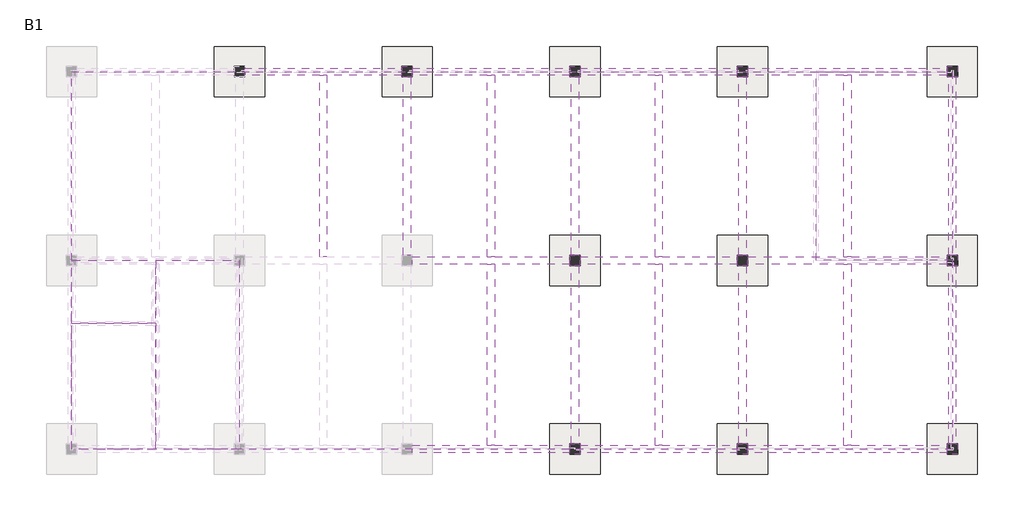
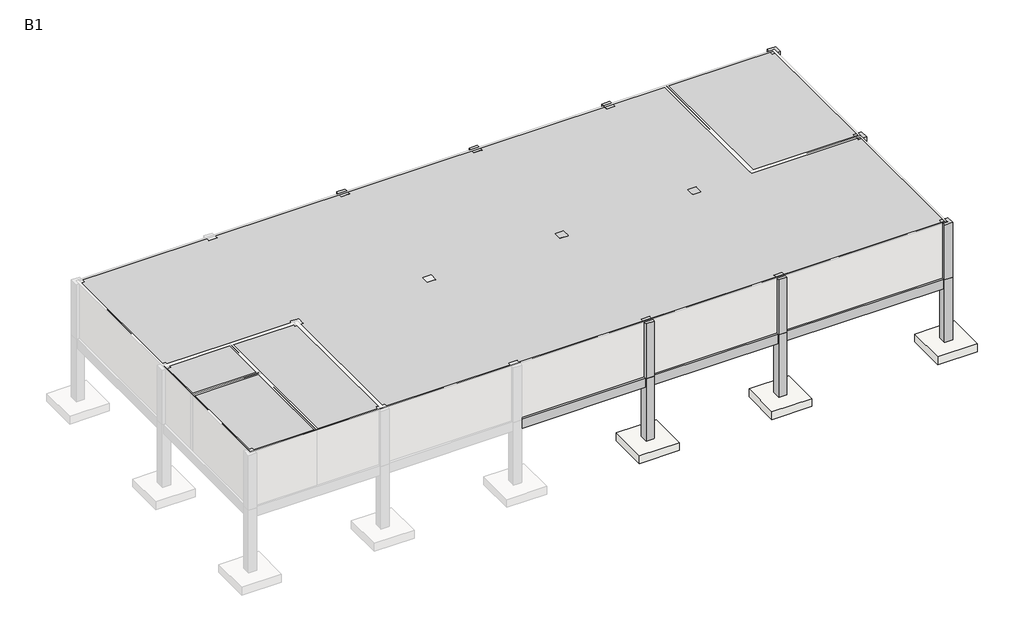
# One storey, part 2 of 2: 24 beams, 21 columns, 11 slabs, 5 proxies.
# Revit data of these elements (continued)
# Element 27 (IfcBuildingElementProxy, "Space Planning Box_hec : Space Planning Box_hec") (continued)
#   Interior Finish = "IW5..N/A..N/A,,WK3..N/A,,FL2..N/A,,N/A..N/A"
#   Exterior Finish = "N/A..N/A,,EW2..N/A..N/A"
#   Department = "AR"
#   ceiling height = 0
#   Width = 4000 mm
#   Program Area = 0.00 m²
#   Length = 9000 mm
#   Height = 3500 mm
#   Area = 36.00 m²
#   Fill Color = Cyan
#   Phase Created = New Construction
#   Materials on its faces: "Cyan"
# Element 28 (IfcBuildingElementProxy, "Space Planning Box_hec : Space Planning Box_hec")
#   Room Name = "Elevator"
#   Interior Finish = "N/A..N/A..N/A,,N/A..N/A,,,,CL3..N/A"
#   Exterior Finish = "N/A..N/A,,EW2..N/A..N/A"
#   Department = "AR"
#   ceiling height = 0
#   Width = 4000 mm
#   Program Area = 0.00 m²
#   Length = 3000 mm
#   Height = 3500 mm
#   Area = 12.00 m²
#   Fill Color = Cyan
#   Phase Created = New Construction
#   Materials on its faces: "Cyan"
# Element 29 (IfcBuildingElementProxy, "Space Planning Box_hec : Space Planning Box_hec")
#   Room Name = "Stairway"
#   Interior Finish = "IW5..N/A..N/A,,WK3..N/A,,FL2..N/A,,CL1..N/A"
#   Exterior Finish = "N/A..N/A,,EW2..N/A..N/A"
#   Department = "PATHV1"
#   ceiling height = 0
#   Width = 4000 mm
#   Program Area = 36.00 m²
#   Length = 6000 mm
#   Height = 3500 mm
#   Area = 24.00 m²
#   Fill Color = Green
#   Phase Created = New Construction
#   Materials on its faces: "Green"
# Elements 30, 31, 32, 33, 34, 35, 36, 37, 38, 39, 40, 41, 42, 43, 44, 45, 46, 47, 48, 49, 50 (IfcColumn, "Concrete-Rectangular-Column : CL111_500x500")
#   Comments = ""
#   hec_material3 = none
#   hec_material2 = none
#   hec_material1 = none
#   Structural Material = 콘크리트 - 현장타설 콘크리트
#   Phase Created = New Construction
#   Materials on its faces: "콘크리트 - 현장타설 콘크리트"
# Elements 51, 52, 53, 54, 55, 56, 57, 58, 59, 60, 61 (IfcSlab, "FT112-Footing-Rectangular : FT112_2400x2400x500")
#   Comments = ""
#   hec_material3 = none
#   hec_material2 = none
#   hec_material1 = none
#   Structural Material = 콘크리트 - 현장타설 콘크리트
#   Phase Created = New Construction
#   Materials on its faces: "콘크리트 - 현장타설 콘크리트"
# Materials
#   "콘크리트 - 현장타설 콘크리트": class "콘크리트", colour RGB 192 192 192, transparency 0
#   "Cyan": class "Generic", colour RGB 0 255 255, transparency 0.2, Cost = 0
#   "A03AE056-00001_Bitumen/Bituminous/Asphalt Coating": class "Generic", colour RGB 17 17 17, transparency 0, Description = "Damp-proofing", W00) Work Master Code = "A03AE056-00001", W01) Work Master_Lv1 = "Concrete Work", W02) Work Master_Lv2 = "Concrete Protective Coating (U/G)", W03) Work Master_Spec.1 = "Bitumen/Bituminous/Asphalt Coating", Cost = 0
#   "A03AC035-00001_Form Work (3 times in use)_Flat": class "Wood", colour RGB 149 120 74, transparency 0, Description = "Plywood", W00) Work Master Code = "A03AC035-00001", W01) Work Master_Lv1 = "Concrete Work", W02) Work Master_Lv2 = "Substructure Work", W03) Work Master_Spec.1 = "Form Work (3 times in use)", W04) Work Master_Spec.2 = "Flat Form", W05) Work Master_Spec.3 = "Dressed Lumber, Plywood or Steel Form(Wood Planks are not Allowed) incl. Chamfer", Cost = 0
#   "A03AC032-00007_Structural Concrete_Type1_25MPa-30Mpa": class "Concrete", colour RGB 176 176 176, transparency 0, Keynote = "09910.A1", Description = "Reinf. Conc.", W00) Work Master Code = "A03AC032-00007", W01) Work Master_Lv1 = "Concrete Work", W02) Work Master_Lv2 = "Substructure Work", W03) Work Master_Spec.1 = "Structural Concrete", W04) Work Master_Spec.2 = "Cement Type-1", W05) Work Master_Spec.3 = "25MPa < F'c (Cylinder Strength) ≤ 30MPa", Cost = 0
#   "Orange": class "Generic", colour RGB 255 165 0, transparency 0.2, Cost = 0
#   "Green": class "Generic", colour RGB 0 128 0, transparency 0.2, Cost = 0
